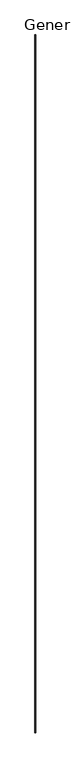
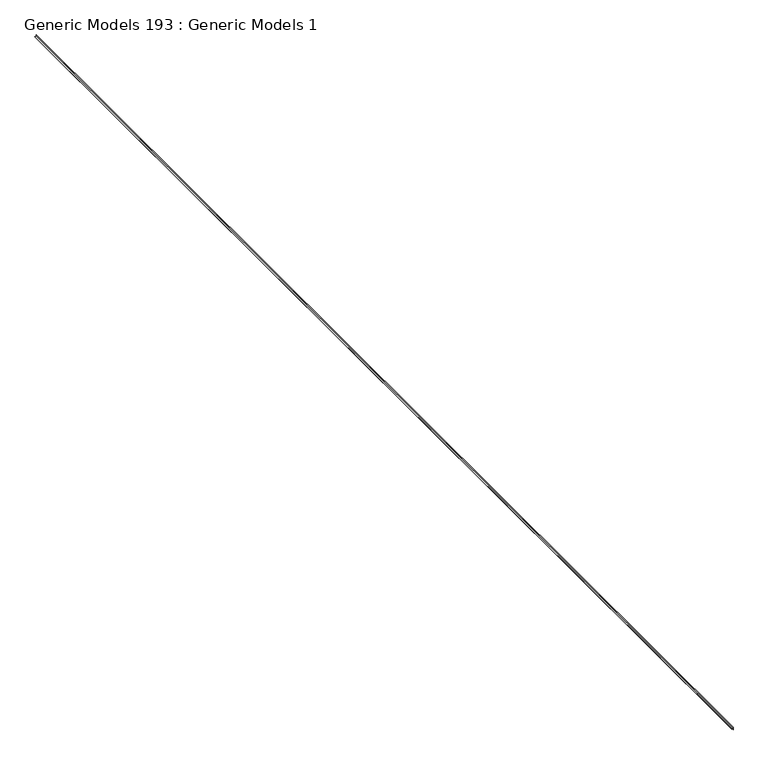
"""IFC4 building model written with IfcOpenShell, lengths in millimetres: proxy geometry, Generic Models 193 : Generic Models 1."""

from ifc_helpers import new_model, si_unit, origin, place, context, project, spatial, faceted_brep, source, transform, mapped, element, save


def generic_models_193_generic_models_1_d058d945(model_context):
    return source(origin(), model_context, "Body", "Brep", [
        faceted_brep([(-8999.7331401, 11981.8769662, 126375.541), (-8999.7331401, 11981.8769662, 126336.171), (-9001.0031401, 11981.8769662, 126336.171), (-9001.0031401, 11981.8769662, 126355.221), (-9020.6881401, 11981.8769662, 126355.221), (-9020.6881401, 11981.8769662, 126351.7412), (-9021.9581401, 11981.8769662, 126351.7412), (-9021.9581401, 11981.8769662, 126356.491), (-9001.0031401, 11981.8769662, 126356.491), (-9001.0031401, 11981.8769662, 126375.541), (-8999.7331401, -7068.1230338, 126375.541), (-9001.0031401, -7068.1230338, 126375.541), (-9001.0031401, -7068.1230338, 126356.491), (-9021.9581401, -7068.1230338, 126356.491), (-9021.9581401, -7068.1230338, 126351.7412), (-9020.6881401, -7068.1230338, 126351.7412), (-9020.6881401, -7068.1230338, 126355.221), (-9001.0031401, -7068.1230338, 126355.221), (-9001.0031401, -7068.1230338, 126336.171), (-8999.7331401, -7068.1230338, 126336.171), (-9021.9581401, 11778.6769662, 126351.7412), (-9021.9581401, -6864.9230338, 126351.7412), (-9020.6881401, 11778.6769662, 126351.7412), (-9020.6881401, -6864.9230338, 126351.7412), (-9020.6881401, 11778.6769662, 126355.221), (-9020.6881401, -6864.9230338, 126355.221)], [[[0, 1, 2, 3, 4, 5, 6, 7, 8, 9]], [[10, 11, 12, 13, 14, 15, 16, 17, 18, 19]], [[0, 9, 11, 10]], [[9, 8, 12, 11]], [[8, 7, 13, 12]], [[7, 6, 20, 21, 14, 13]], [[6, 5, 22, 23, 15, 14, 21, 20]], [[5, 4, 24, 25, 16, 15, 23, 22]], [[4, 3, 17, 16, 25, 24]], [[3, 2, 18, 17]], [[2, 1, 19, 18]], [[1, 0, 10, 19]]]),
    ])


if __name__ == "__main__":
    model = new_model("IFC4")
    model_context = context("Model", 3, world=origin())
    ifc_project = project(units=[si_unit("LENGTHUNIT", "METRE", prefix="MILLI")], contexts=[model_context])
    site = spatial("IfcSite", under=ifc_project)
    building = spatial("IfcBuilding", under=site)
    placement = place(None, origin())
    generic_models_193_generic_models_1_shape = generic_models_193_generic_models_1_d058d945(model_context)
    element("IfcBuildingElementProxy", 1, Name="Generic Models 193 : Generic Models 1", ObjectType="Generic Models 193 : Generic Models 1", at=placement, inside=building, context=model_context, shape_type="MappedRepresentation", body=[
        mapped(generic_models_193_generic_models_1_shape, transform((0.0, 0.0, 0.0), x_axis=(1.0, 0.0, 0.0), y_axis=(0.0, 1.0, 0.0), z_axis=(0.0, 0.0, 1.0))),
    ])
    save(model, "model.ifc")

# Revit data of these elements
# Element 1 (IfcBuildingElementProxy, "Generic Models 193 : Generic Models 1")
#   Materials on its faces: "_ 16 GA. COPPER VENTED T REVEAL BEAD (CONT. AROUND PERIMETER OF BEAM)"
# Materials
#   "_ 16 GA. COPPER VENTED T REVEAL BEAD (CONT. AROUND PERIMETER OF BEAM)": class "Generic", colour RGB 253 192 103, transparency 0, Cost = 0
